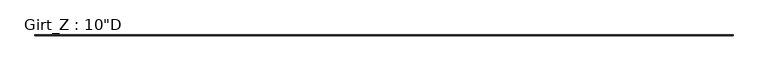
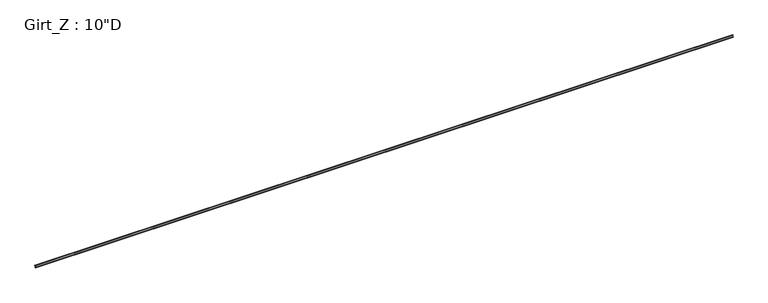
"""IFC4 building model written with IfcOpenShell, lengths in millimetres: beam geometry."""

import ifcopenshell
import ifcopenshell.guid

model = None  # the IFC model being written
_history = None  # IfcOwnerHistory: only IFC2X3 demands one
_inside = {}  # id of a spatial element -> (the spatial element, [elements in it])
_under = {}  # id of a project, library or spatial element -> (it, [spatial elements below it])
_declared = {}  # id of a project -> (the project, [libraries it declares])
_typed = {}  # id of a type object -> (the type object, [elements of that type])
_made_of = {}  # id of a material, layer set ... -> (it, [elements and type objects made of it])


def new_model(schema):
    """Start an empty IFC model of exactly this schema.

    Asked for "IFC4X3", IfcOpenShell would pick the latest addendum, in which some entities
    have other attributes; the version numbers below select the first issue.
    IFC2X3 requires an IfcOwnerHistory on every rooted entity: one is made here for all.
    """
    global model, _history
    if schema == "IFC4X3":
        model = ifcopenshell.file(schema_version=(4, 3, 0, 0))
    else:
        model = ifcopenshell.file(schema=schema)
    _inside.clear()
    _under.clear()
    _declared.clear()
    _typed.clear()
    _made_of.clear()
    _history = None
    if model.schema == "IFC2X3":
        org = make("IfcOrganization", Name="unknown")
        user = make(
            "IfcPersonAndOrganization",
            ThePerson=make("IfcPerson", FamilyName="unknown"),
            TheOrganization=org,
        )
        app = make(
            "IfcApplication",
            ApplicationDeveloper=org,
            Version="unknown",
            ApplicationFullName="unknown",
            ApplicationIdentifier="unknown",
        )
        _history = make(
            "IfcOwnerHistory",
            OwningUser=user,
            OwningApplication=app,
            ChangeAction="ADDED",
            CreationDate=0,
        )
    return model


def make(cls, **values):
    """One entity of the class cls with the attributes given. An attribute that is None is left unset."""
    return model.create_entity(
        cls, **{name: value for name, value in values.items() if value is not None}
    )


def rooted(cls, **values):
    """An entity with a GlobalId (a new one), such as an element, a storey or a relation."""
    return make(cls, GlobalId=ifcopenshell.guid.new(), OwnerHistory=_history, **values)


def si_unit(unit_type, name, prefix=None):
    """IfcSIUnit, for example si_unit("LENGTHUNIT", "METRE", prefix="MILLI")."""
    return make("IfcSIUnit", UnitType=unit_type, Prefix=prefix, Name=name)


def assignment(units):
    """IfcUnitAssignment: the units of a project."""
    return None if units is None else make("IfcUnitAssignment", Units=units)


def point(xyz):
    """IfcCartesianPoint."""
    return None if xyz is None else make("IfcCartesianPoint", Coordinates=xyz)


def direction(xyz):
    """IfcDirection."""
    return None if xyz is None else make("IfcDirection", DirectionRatios=xyz)


def frame(location, z_axis=None, x_axis=None):
    """IfcAxis2Placement3D, a coordinate frame: its origin and axes. An axis left out is left unset."""
    return make(
        "IfcAxis2Placement3D",
        Location=point(location),
        Axis=direction(z_axis),
        RefDirection=direction(x_axis),
    )


def frame_2d(location, x_axis=None):
    """IfcAxis2Placement2D, a coordinate frame in the plane: its origin and x axis."""
    return make(
        "IfcAxis2Placement2D", Location=point(location), RefDirection=direction(x_axis)
    )


def origin():
    """The frame at (0, 0, 0) with its axes left unset."""
    return frame((0.0, 0.0, 0.0))


def place(relative_to, where):
    """IfcLocalPlacement: puts the frame where relative to a parent placement (None: the world)."""
    return make(
        "IfcLocalPlacement", PlacementRelTo=relative_to, RelativePlacement=where
    )


def context(
    kind, dimensions, precision=None, world=None, true_north=None, identifier=None
):
    """IfcGeometricRepresentationContext, for example the 3D "Model" context."""
    return make(
        "IfcGeometricRepresentationContext",
        ContextIdentifier=identifier,
        ContextType=kind,
        CoordinateSpaceDimension=dimensions,
        Precision=precision,
        WorldCoordinateSystem=world,
        TrueNorth=true_north,
    )


def project(units=None, contexts=None):
    """IfcProject with its units and contexts."""
    return rooted(
        "IfcProject",
        Name="project",
        RepresentationContexts=contexts,
        UnitsInContext=assignment(units),
    )


def spatial(cls, under=None, at=None, **own):
    """A site, building, storey or space (cls), placed at a placement, below another one or the project."""
    s = rooted(cls, ObjectPlacement=at, **own)
    if under is not None:
        _under.setdefault(under.id(), (under, []))[1].append(s)
    return s


def polyline(points):
    """IfcPolyline through the points."""
    return make("IfcPolyline", Points=[point(p) for p in points])


def circle_curve(where, radius):
    """IfcCircle in the frame where."""
    return make("IfcCircle", Position=where, Radius=radius)


def trimmed(basis, trim1, trim2, sense, master):
    """IfcTrimmedCurve: the piece of a basis curve between two trims."""
    return make(
        "IfcTrimmedCurve",
        BasisCurve=basis,
        Trim1=trim1,
        Trim2=trim2,
        SenseAgreement=sense,
        MasterRepresentation=master,
    )


def segment(curve, same_sense, transition):
    """IfcCompositeCurveSegment."""
    return make(
        "IfcCompositeCurveSegment",
        Transition=transition,
        SameSense=same_sense,
        ParentCurve=curve,
    )


def composite_curve(segments, self_intersect=None):
    """IfcCompositeCurve: segments joined end to end."""
    return make("IfcCompositeCurve", Segments=segments, SelfIntersect=self_intersect)


def outline(outer, holes=None, kind="AREA"):
    """IfcArbitraryClosedProfileDef: a profile drawn as a closed curve; with holes, ...WithVoids."""
    if holes is None:
        return make("IfcArbitraryClosedProfileDef", ProfileType=kind, OuterCurve=outer)
    return make(
        "IfcArbitraryProfileDefWithVoids",
        ProfileType=kind,
        OuterCurve=outer,
        InnerCurves=holes,
    )


def extrude(swept, where, along, depth):
    """IfcExtrudedAreaSolid: the profile swept, set in the frame where, extruded along a direction by depth."""
    return make(
        "IfcExtrudedAreaSolid",
        SweptArea=swept,
        Position=where,
        ExtrudedDirection=direction(along),
        Depth=depth,
    )


def shape(context_of_items, identifier, shape_type, items):
    """IfcShapeRepresentation: the items that make up one representation, for example the "Body"."""
    return make(
        "IfcShapeRepresentation",
        ContextOfItems=context_of_items,
        RepresentationIdentifier=identifier,
        RepresentationType=shape_type,
        Items=items,
    )


def source(mapping_origin, context_of_items, identifier, shape_type, items):
    """IfcRepresentationMap: a shape defined once, which mapped items show again and again."""
    return make(
        "IfcRepresentationMap",
        MappingOrigin=mapping_origin,
        MappedRepresentation=shape(context_of_items, identifier, shape_type, items),
    )


def transform(
    local_origin,
    x_axis=None,
    y_axis=None,
    z_axis=None,
    scale=None,
    scale2=None,
    scale3=None,
    uniform=True,
):
    """IfcCartesianTransformationOperator3D, or its non-uniform kind. x_axis, y_axis, z_axis: its Axis1, 2, 3."""
    if uniform:
        return make(
            "IfcCartesianTransformationOperator3D",
            Axis1=direction(x_axis),
            Axis2=direction(y_axis),
            LocalOrigin=point(local_origin),
            Scale=scale,
            Axis3=direction(z_axis),
        )
    return make(
        "IfcCartesianTransformationOperator3DnonUniform",
        Axis1=direction(x_axis),
        Axis2=direction(y_axis),
        LocalOrigin=point(local_origin),
        Scale=scale,
        Axis3=direction(z_axis),
        Scale2=scale2,
        Scale3=scale3,
    )


def mapped(mapping_source, mapping_target):
    """IfcMappedItem: shows the shape of a source again, moved by a transform."""
    return make(
        "IfcMappedItem", MappingSource=mapping_source, MappingTarget=mapping_target
    )


def made_of(thing, what):
    """Note that an element or type object is made of a material, layer set ...; save() writes the relation."""
    if what is not None:
        _made_of.setdefault(what.id(), (what, []))[1].append(thing)
    return thing


def element(
    cls,
    number,
    at=None,
    inside=None,
    cuts=None,
    type_object=None,
    material=None,
    context=None,
    identifier="Body",
    shape_type=None,
    held_by="IfcProductDefinitionShape",
    body=None,
    shapes=None,
    **own,
):
    """One element of the class cls, such as IfcWall. Its Tag is "e" and its number.

    at: its placement. inside: the storey or other place that contains it. cuts: it is an
    opening in that element (IfcRelVoidsElement). A single representation is given by context,
    identifier, shape_type and body (its items); several are given by shapes. held_by: the class
    of the entity that holds the representations. save() writes the other relations.
    """
    e = rooted(cls, Tag="e%d" % number, ObjectPlacement=at, **own)
    if body is not None:
        shapes = [shape(context, identifier, shape_type, body)]
    if shapes is not None:
        e.Representation = make(held_by, Representations=shapes)
    if inside is not None:
        _inside.setdefault(inside.id(), (inside, []))[1].append(e)
    if cuts is not None:
        rooted(
            "IfcRelVoidsElement", RelatingBuildingElement=cuts, RelatedOpeningElement=e
        )
    if type_object is not None:
        _typed.setdefault(type_object.id(), (type_object, []))[1].append(e)
    return made_of(e, material)


def aggregate(whole, parts):
    """IfcRelAggregates: a whole, such as a stair, and the parts it consists of."""
    return rooted("IfcRelAggregates", RelatingObject=whole, RelatedObjects=parts)


def save(model, path):
    """Write the relations noted so far, then the file.

    IfcRelAggregates (storeys below a building ...), IfcRelContainedInSpatialStructure (elements
    in a storey), IfcRelDefinesByType, IfcRelAssociatesMaterial and IfcRelDeclares: one each for
    every whole, place, type object, material and project.
    """
    for whole, parts in _under.values():
        aggregate(whole, parts)
    for where, things in _inside.values():
        rooted(
            "IfcRelContainedInSpatialStructure",
            RelatedElements=things,
            RelatingStructure=where,
        )
    for kind, things in _typed.values():
        rooted("IfcRelDefinesByType", RelatedObjects=things, RelatingType=kind)
    for what, things in _made_of.values():
        rooted("IfcRelAssociatesMaterial", RelatedObjects=things, RelatingMaterial=what)
    for by, libraries in _declared.values():
        rooted("IfcRelDeclares", RelatingContext=by, RelatedDefinitions=libraries)
    model.write(path)


def beam_affa7a5f(model_context):
    return source(origin(), model_context, "Body", "SweptSolid", [
        extrude(outline(composite_curve([segment(polyline([(63.5, 127.0), (75.745104, 112.4068534), (73.6169367, 110.621109), (62.204539, 124.221875), (3.3005807, 124.221875)]), True, "CONTINUOUS"), segment(trimmed(circle_curve(frame_2d((3.3741066, 122.2381931)), 1.9850441), [point((3.3005807, 124.221875))], [point((1.3890625, 122.2381931))], True, "CARTESIAN"), True, "CONTINUOUS"), segment(polyline([(1.3890625, 122.2381931), (1.3890625, -122.2375)]), True, "CONTINUOUS"), segment(trimmed(circle_curve(frame_2d((-3.3734375, -122.2375)), 4.7625), [point((1.3890625, -122.2375))], [point((-3.3734375, -127.0))], False, "CARTESIAN"), True, "CONTINUOUS"), segment(polyline([(-3.3734375, -127.0), (-63.5, -127.0), (-75.745104, -112.4068534), (-73.6169367, -110.621109), (-62.204539, -124.221875), (-3.2694106, -124.221875)]), True, "CONTINUOUS"), segment(trimmed(circle_curve(frame_2d((-3.3748024, -122.2389339)), 1.9857399), [point((-3.2694106, -124.221875))], [point((-1.3890625, -122.2389339))], True, "CARTESIAN"), True, "CONTINUOUS"), segment(polyline([(-1.3890625, -122.2389339), (-1.3890625, 122.2375)]), True, "CONTINUOUS"), segment(trimmed(circle_curve(frame_2d((3.3734375, 122.2375)), 4.7625), [point((-1.3890625, 122.2375))], [point((3.3734375, 127.0))], False, "CARTESIAN"), True, "CONTINUOUS"), segment(polyline([(3.3734375, 127.0), (63.5, 127.0)]), True, "CONTINUOUS")], self_intersect=False)), frame((-51384.2, 0.0, 0.0), z_axis=(1.0, 0.0, 0.0), x_axis=(0.0, 1.0, 0.0)), (0.0, 0.0, 1.0), 102679.5),
    ])


if __name__ == "__main__":
    model = new_model("IFC4")
    model_context = context("Model", 3, world=origin())
    ifc_project = project(units=[si_unit("LENGTHUNIT", "METRE", prefix="MILLI")], contexts=[model_context])
    site = spatial("IfcSite", under=ifc_project)
    building = spatial("IfcBuilding", under=site)
    placement = place(None, origin())
    beam_shape = beam_affa7a5f(model_context)
    element("IfcBeam", 1, ObjectType="Girt_Z : 10\"D", at=placement, inside=building, context=model_context, shape_type="MappedRepresentation", body=[
        mapped(beam_shape, transform((0.0, 0.0, 0.0), x_axis=(1.0, 0.0, 0.0), y_axis=(0.0, 1.0, 0.0), z_axis=(0.0, 0.0, 1.0))),
    ])
    save(model, "model.ifc")

# Revit data of these elements
# Type "Girt_Z : 10\"D"
#   Web_Thickness = 0' - 0 7/64"
#   Length [instance default] = 10' - 0"
#   Leg_1 = 0' - 2 1/2"
#   Height = 0' - 10"
#   Structural Material [instance default] = none
